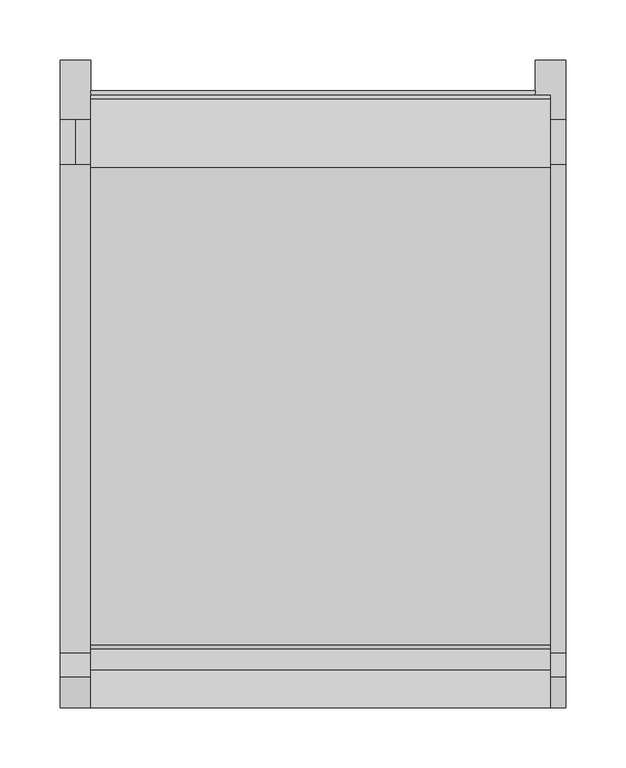
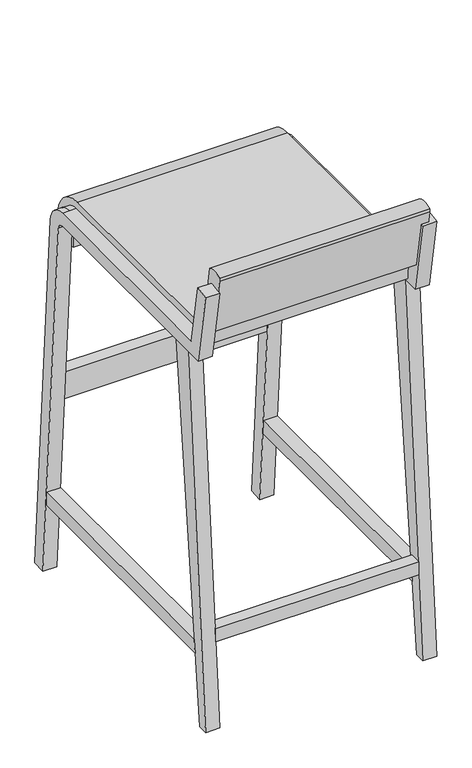
"""IFC4 building model written with IfcOpenShell, lengths in millimetres: furniture geometry, Bar_Stool_6722[1] : Bar_Stool_6722[1]."""

from ifc_helpers import new_model, si_unit, point, frame, frame_2d, origin, place, context, project, spatial, polyline, circle_curve, trimmed, segment, composite_curve, outline, extrude, source, transform, mapped, element, save
from ifc_brep_helpers import plane_surface, cylinder_surface, revolved_surface, advanced_brep


def furniture_d221970b(model_context):
    return source(origin(), model_context, "Body", "SolidModel", [
        advanced_brep(
        [(419.1, 25.0141169, 838.4759165), (393.7, 25.0141169, 838.4759165), (393.7, 0.0, 834.0652528), (419.1, 0.0, 834.0652528), (419.1, 45.2169423, 723.9), (393.7, 45.2169423, 723.9), (393.7, 450.0350637, 723.9), (393.7, 488.0397183, 688.4937383), (393.7, 536.7759384, 0.8979128), (393.7, 511.439502, -0.8979128), (393.7, 462.7032819, 686.6979128), (393.7, 450.0350637, 698.5), (393.7, 23.9038117, 698.5), (419.1, 23.9038117, 698.5), (419.1, 450.0350637, 698.5), (419.1, 462.7032819, 686.6979128), (419.1, 511.439502, -0.8979128), (419.1, 536.7759384, 0.8979128), (419.1, 488.0397183, 688.4937383), (419.1, 450.0350637, 723.9), (406.4, 450.0350637, 723.9), (406.4, 488.0397183, 688.4937383)],
        [
            (0, 1),
            (1, 2),
            (2, 3),
            (3, 0),
            (0, 4),
            (4, 5),
            (5, 1),
            (5, 6),
            (6, 7, circle_curve(frame((393.7, 450.0350637, 685.8), z_axis=(-1.0, 0.0, 0.0), x_axis=(0.0, 0.0, 1.0)), 38.1)),
            (7, 8),
            (8, 9),
            (9, 10),
            (10, 11, circle_curve(frame((393.7, 450.0350637, 685.8), z_axis=(1.0, 0.0, 0.0), x_axis=(0.0, 0.0, 1.0)), 12.7)),
            (11, 12),
            (12, 2),
            (12, 13),
            (13, 3),
            (13, 14),
            (14, 15, circle_curve(frame((419.1, 450.0350637, 685.8), z_axis=(-1.0, 0.0, 0.0), x_axis=(0.0, 0.0, 1.0)), 12.7)),
            (15, 16),
            (16, 17),
            (17, 18),
            (18, 19, circle_curve(frame((419.1, 450.0350637, 685.8), z_axis=(1.0, 0.0, 0.0), x_axis=(0.0, 0.0, 1.0)), 38.1)),
            (19, 4),
            (19, 20),
            (20, 6),
            (11, 14),
            (21, 20, circle_curve(frame((406.4, 450.0350637, 685.8), z_axis=(1.0, 0.0, 0.0), x_axis=(0.0, 0.0, 1.0)), 38.1)),
            (18, 21),
            (21, 7),
            (10, 15),
            (17, 8),
            (9, 16),
        ],
        [
            plane_surface(frame((406.4, 12.5070585, 836.2705846), z_axis=(0.0, -0.17364817766692853, 0.9848077530122085), x_axis=(1.0, 0.0, 0.0))),
            plane_surface(frame((406.4, 25.0141169, 838.4759165), z_axis=(0.0, 0.9848077530122085, 0.17364817766692814), x_axis=(0.0, 0.17364817766692814, -0.9848077530122085))),
            plane_surface(frame((393.7, 25.0141169, 838.4759165), z_axis=(-1.0, 0.0, 0.0), x_axis=(0.0, 0.17364817766692808, -0.9848077530122085))),
            plane_surface(frame((393.7, 0.0, 834.0652528), z_axis=(0.0, -0.9848077530122085, -0.17364817766692817), x_axis=(0.0, 0.17364817766692817, -0.9848077530122085))),
            plane_surface(frame((419.1, 0.0, 834.0652528), z_axis=(1.0000000000000002, 0.0, 0.0), x_axis=(0.0, 0.1736481776669284, -0.9848077530122085))),
            plane_surface(frame((406.4, 45.2169423, 723.9), z_axis=(0.0, 0.0, 1.0), x_axis=(0.0, 1.0, 0.0))),
            plane_surface(frame((393.7, 23.9038117, 698.5), z_axis=(0.0, 0.0, -1.0), x_axis=(0.0, 1.0, 0.0))),
            cylinder_surface(frame((406.4, 450.0350637, 685.8), z_axis=(-1.0, 0.0, 0.0), x_axis=(0.0, 0.0, 1.0)), 38.1),
            revolved_surface(polyline([(393.7, 450.0350637, 698.5), (419.1, 450.0350637, 698.5)]), (406.4, 450.0350637, 685.8), (-1.0, 0.0, 0.0)),
            plane_surface(frame((406.4, 488.0397183, 688.4937383), z_axis=(0.0, 0.9974974969901172, 0.07070179275273744), x_axis=(0.0, 0.07070179275273744, -0.9974974969901172))),
            plane_surface(frame((393.7, 462.7032819, 686.6979128), z_axis=(0.0, -0.9974974969901172, -0.07070179275273743), x_axis=(0.0, 0.07070179275273743, -0.9974974969901172))),
            plane_surface(frame((406.4, 524.1077202, 0.0), z_axis=(0.0, 0.07070179275273399, -0.9974974969901175), x_axis=(1.0, 0.0, 0.0))),
        ],
        [
            (0, [[1, 2, 3, 4]]),
            (1, [[5, 6, 7, -1]]),
            (2, [[-2, -7, 8, 9, 10, 11, 12, 13, 14, 15]]),
            (3, [[-3, -15, 16, 17]]),
            (4, [[-4, -17, 18, 19, 20, 21, 22, 23, 24, -5]]),
            (5, [[-6, -24, 25, 26, -8]]),
            (6, [[-16, -14, 27, -18]]),
            (7, [[28, -25, -23, 29]]),
            (7, [[-9, -26, -28, 30]]),
            (8, [[-19, -27, -13, 31]]),
            (9, [[-10, -30, -29, -22, 32]]),
            (10, [[-20, -31, -12, 33]]),
            (11, [[-32, -21, -33, -11]]),
        ],
    ),
        extrude(outline(composite_curve([segment(polyline([(48.4096386, 756.5644068), (44.0710693, 752.2258375), (19.1416957, 748.2774126), (0.0, 856.8353632), (0.0, 863.1853632)]), True, "CONTINUOUS"), segment(trimmed(circle_curve(frame_2d((15.7612691, 828.3540875)), 38.2313401), [point((0.0, 863.1853632))], [point((31.5225381, 863.1853632))], False, "CARTESIAN"), True, "CONTINUOUS"), segment(polyline([(31.5225381, 863.1853632), (48.4096386, 756.5644068)]), True, "CONTINUOUS")], self_intersect=False)), frame((25.4, 0.0, 0.0), z_axis=(1.0, 0.0, 0.0), x_axis=(0.0, 1.0, 0.0)), (0.0, 0.0, 1.0), 381.0),
        extrude(outline(composite_curve([segment(polyline([(51.6744261, 737.5144068), (447.8968201, 737.5144068)]), True, "CONTINUOUS"), segment(trimmed(circle_curve(frame_2d((447.8968201, 676.6245275)), 60.8898793), [point((447.8968201, 737.5144068))], [point((505.1145904, 697.4500928))], False, "CARTESIAN"), True, "CONTINUOUS"), segment(trimmed(circle_curve(frame_2d((460.5585493, 681.23302)), 47.4155486), [point((505.1145904, 697.4500928))], [point((484.2663236, 640.1699505))], False, "CARTESIAN"), True, "CONTINUOUS"), segment(polyline([(484.2663236, 640.1699505), (460.5585493, 643.13302), (460.5585493, 681.23302), (452.817441, 704.85), (46.417441, 704.85), (43.9498561, 733.0546243), (51.6744261, 737.5144068)]), True, "CONTINUOUS")], self_intersect=False)), frame((25.4, 0.0, 0.0), z_axis=(1.0, 0.0, 0.0), x_axis=(0.0, 1.0, 0.0)), (0.0, 0.0, 1.0), 381.0),
        extrude(outline(polyline([(393.7, 11.6871233), (25.4, 11.6871233), (25.4, 33.1441574), (393.7, 33.1441574), (393.7, 11.6871233)])), frame((0.0, 0.0, 157.9619127), z_axis=(0.0, 0.0, 1.0), x_axis=(1.0, 0.0, 0.0)), (0.0, 0.0, 1.0), 25.4),
        extrude(outline(polyline([(393.7, 488.2695397), (25.4, 488.2695397), (25.4, 511.439502), (393.7, 511.439502), (393.7, 488.2695397)])), frame((0.0, 0.0, 335.7619127), z_axis=(0.0, 0.0, 1.0), x_axis=(1.0, 0.0, 0.0)), (0.0, 0.0, 1.0), 50.8),
        extrude(outline(polyline([(500.1796497, 157.9619127), (500.1796497, 132.5619127), (32.9828185, 132.5619127), (35.652466, 157.9619127), (500.1796497, 157.9619127)])), frame((393.7, 0.0, 0.0), z_axis=(1.0, 0.0, 0.0), x_axis=(0.0, 1.0, 0.0)), (0.0, 0.0, 1.0), 25.4),
        extrude(outline(polyline([(500.1796497, 157.9619127), (500.1796497, 132.5619127), (32.9828185, 132.5619127), (35.652466, 157.9619127), (500.1796497, 157.9619127)])), frame((0.0, 0.0, 0.0), z_axis=(1.0, 0.0, 0.0), x_axis=(0.0, 1.0, 0.0)), (0.0, 0.0, 1.0), 25.4),
        extrude(outline(polyline([(0.0, 0.0), (55.3031462, 698.5), (92.4653083, 698.5), (19.05, 0.0), (0.0, 0.0)])), frame((393.7, 0.0, 0.0), z_axis=(1.0, 0.0, 0.0), x_axis=(0.0, 1.0, 0.0)), (0.0, 0.0, 1.0), 25.4),
        advanced_brep(
        [(25.4, 25.0141169, 838.4759165), (0.0, 25.0141169, 838.4759165), (0.0, 0.0, 834.0652528), (25.4, 0.0, 834.0652528), (25.4, 45.2169423, 723.9), (0.0, 45.2169423, 723.9), (0.0, 450.0350637, 723.9), (0.0, 488.0397183, 688.4937383), (0.0, 536.7759384, 0.8979128), (0.0, 511.439502, -0.8979128), (0.0, 462.7032819, 686.6979128), (0.0, 450.0350637, 698.5), (0.0, 23.9038117, 698.5), (25.4, 23.9038117, 698.5), (25.4, 450.0350637, 698.5), (25.4, 462.7032819, 686.6979128), (25.4, 511.439502, -0.8979128), (25.4, 536.7759384, 0.8979128), (25.4, 488.0397183, 688.4937383), (25.4, 450.0350637, 723.9), (12.7, 450.0350637, 723.9), (12.7, 488.0397183, 688.4937383)],
        [
            (0, 1),
            (1, 2),
            (2, 3),
            (3, 0),
            (0, 4),
            (4, 5),
            (5, 1),
            (5, 6),
            (6, 7, circle_curve(frame((0.0, 450.0350637, 685.8), z_axis=(-1.0, 0.0, 0.0), x_axis=(0.0, 0.0, 1.0)), 38.1)),
            (7, 8),
            (8, 9),
            (9, 10),
            (10, 11, circle_curve(frame((0.0, 450.0350637, 685.8), z_axis=(1.0, 0.0, 0.0), x_axis=(0.0, 0.0, 1.0)), 12.7)),
            (11, 12),
            (12, 2),
            (12, 13),
            (13, 3),
            (13, 14),
            (14, 15, circle_curve(frame((25.4, 450.0350637, 685.8), z_axis=(-1.0, 0.0, 0.0), x_axis=(0.0, 0.0, 1.0)), 12.7)),
            (15, 16),
            (16, 17),
            (17, 18),
            (18, 19, circle_curve(frame((25.4, 450.0350637, 685.8), z_axis=(1.0, 0.0, 0.0), x_axis=(0.0, 0.0, 1.0)), 38.1)),
            (19, 4),
            (19, 20),
            (20, 6),
            (11, 14),
            (7, 21),
            (21, 18),
            (17, 8),
            (15, 10),
            (9, 16),
            (21, 20, circle_curve(frame((12.7, 450.0350637, 685.8), z_axis=(1.0, 0.0, 0.0), x_axis=(0.0, 0.0, 1.0)), 38.1)),
        ],
        [
            plane_surface(frame((12.7, 12.5070585, 836.2705846), z_axis=(0.0, -0.17364817766692853, 0.9848077530122085), x_axis=(1.0, 0.0, 0.0))),
            plane_surface(frame((12.7, 25.0141169, 838.4759165), z_axis=(0.0, 0.9848077530122085, 0.173648177666928), x_axis=(0.0, 0.173648177666928, -0.9848077530122085))),
            plane_surface(frame((0.0, 25.0141169, 838.4759165), z_axis=(-1.0, 0.0, 0.0), x_axis=(0.0, 0.17364817766692875, -0.9848077530122084))),
            plane_surface(frame((0.0, 0.0, 834.0652528), z_axis=(0.0, -0.9848077530122084, -0.17364817766692883), x_axis=(0.0, 0.17364817766692883, -0.9848077530122084))),
            plane_surface(frame((25.4, 0.0, 834.0652528), z_axis=(1.0000000000000002, 0.0, 0.0), x_axis=(0.0, 0.1736481776669284, -0.9848077530122085))),
            plane_surface(frame((12.7, 45.2169423, 723.9), z_axis=(0.0, 0.0, 1.0), x_axis=(0.0, 1.0, 0.0))),
            plane_surface(frame((0.0, 23.9038117, 698.5), z_axis=(0.0, 0.0, -1.0), x_axis=(0.0, 1.0, 0.0))),
            plane_surface(frame((12.7, 488.0397183, 688.4937383), z_axis=(0.0, 0.9974974969901172, 0.07070179275273744), x_axis=(0.0, 0.07070179275273744, -0.9974974969901172))),
            plane_surface(frame((0.0, 462.7032819, 686.6979128), z_axis=(0.0, -0.9974974969901172, -0.07070179275273743), x_axis=(0.0, 0.07070179275273743, -0.9974974969901172))),
            plane_surface(frame((12.7, 524.1077202, 0.0), z_axis=(0.0, 0.07070179275273399, -0.9974974969901175), x_axis=(1.0, 0.0, 0.0))),
            cylinder_surface(frame((12.7, 450.0350637, 685.8), z_axis=(-1.0, 0.0, 0.0), x_axis=(0.0, 0.0, 1.0)), 38.1),
            revolved_surface(polyline([(0.0, 450.0350637, 698.5), (25.4, 450.0350637, 698.5)]), (12.7, 450.0350637, 685.8), (-1.0, 0.0, 0.0)),
        ],
        [
            (0, [[1, 2, 3, 4]]),
            (1, [[5, 6, 7, -1]]),
            (2, [[-2, -7, 8, 9, 10, 11, 12, 13, 14, 15]]),
            (3, [[-3, -15, 16, 17]]),
            (4, [[-4, -17, 18, 19, 20, 21, 22, 23, 24, -5]]),
            (5, [[-6, -24, 25, 26, -8]]),
            (6, [[-16, -14, 27, -18]]),
            (7, [[-10, 28, 29, -22, 30]]),
            (8, [[-20, 31, -12, 32]]),
            (9, [[-30, -21, -32, -11]]),
            (10, [[33, -25, -23, -29]]),
            (10, [[-9, -26, -33, -28]]),
            (11, [[-19, -27, -13, -31]]),
        ],
    ),
        extrude(outline(polyline([(0.0, 0.0), (55.3031462, 698.5), (92.4653083, 698.5), (19.05, 0.0), (0.0, 0.0)])), frame((0.0, 0.0, 0.0), z_axis=(1.0, 0.0, 0.0), x_axis=(0.0, 1.0, 0.0)), (0.0, 0.0, 1.0), 25.4),
    ])


if __name__ == "__main__":
    model = new_model("IFC4")
    model_context = context("Model", 3, world=origin())
    ifc_project = project(units=[si_unit("LENGTHUNIT", "METRE", prefix="MILLI")], contexts=[model_context])
    site = spatial("IfcSite", under=ifc_project)
    building = spatial("IfcBuilding", under=site)
    placement = place(None, origin())
    furniture_shape = furniture_d221970b(model_context)
    element("IfcFurniture", 1, ObjectType="Bar_Stool_6722[1] : Bar_Stool_6722[1]", at=placement, inside=building, context=model_context, shape_type="MappedRepresentation", body=[
        mapped(furniture_shape, transform((0.0, 0.0, 0.0), x_axis=(1.0, 0.0, 0.0), y_axis=(0.0, 1.0, 0.0), z_axis=(0.0, 0.0, 1.0))),
    ])
    save(model, "model.ifc")

# Revit data of these elements
# Type "Bar_Stool_6722[1] : Bar_Stool_6722[1]"
#   Seat = fab
#   Chair Legs = MET
# Element 1 (IfcFurniture, "Bar_Stool_6722[1] : Bar_Stool_6722[1]")
#   Materials on its faces: "MET", "fab"
# Materials
#   "fab": class "Leather", colour RGB 99 104 100, transparency 0
#   "MET": class "Metal", colour RGB 189 187 185, transparency 0
